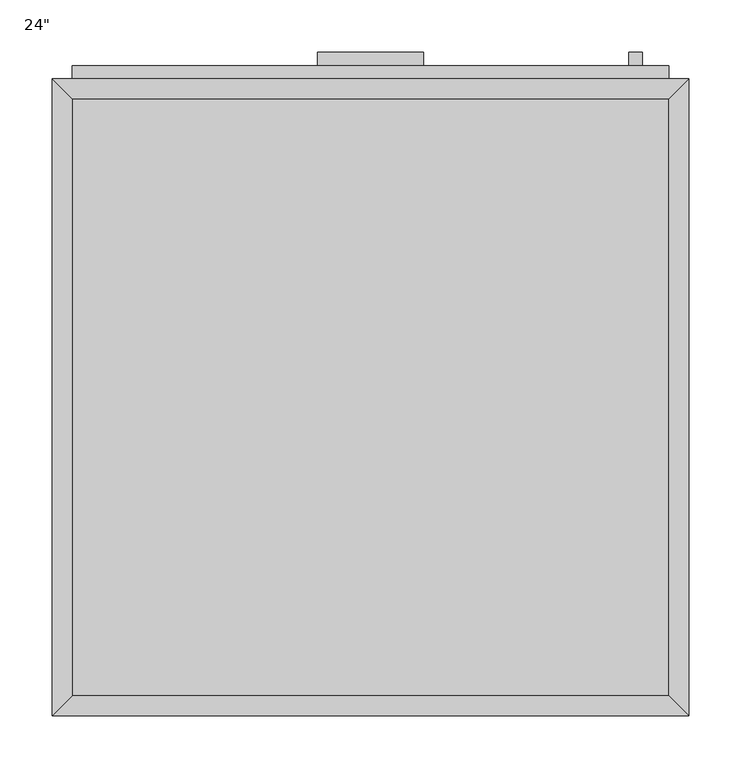
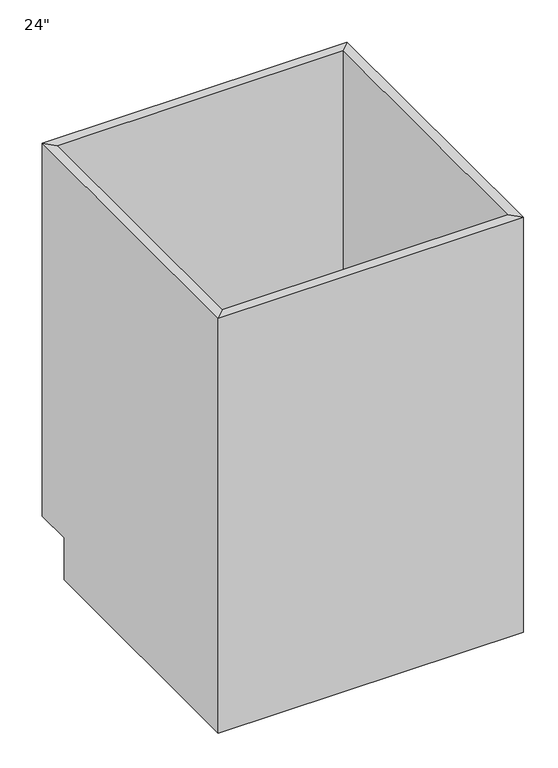
"""IFC4 building model written with IfcOpenShell, lengths in millimetres: furniture geometry."""

from ifc_helpers import new_model, si_unit, frame, origin, place, context, project, spatial, polyline, outline, extrude, faceted_brep, source, transform, mapped, element, save


def furniture_94ff1b7c(model_context):
    return source(origin(), model_context, "Body", "SolidModel", [
        faceted_brep([(304.4877049, 590.55, 876.3), (-267.0122951, 590.55, 876.3), (-267.0122951, 590.55, 88.9), (304.4877049, 590.55, 88.9), (323.5377049, 609.6, 876.3), (-286.0622951, 609.6, 876.3), (323.5377049, 609.6, 88.9), (-286.0622951, 609.6, 88.9), (-267.0122951, 19.05, 876.3), (-267.0122951, 19.05, 88.9), (-267.0122951, 533.4, 88.9), (-286.0622951, 0.0, 876.3), (-286.0622951, 533.4, 88.9), (-286.0622951, 533.4, 0.0), (-286.0622951, 0.0, 0.0), (304.4877049, 19.05, 876.3), (304.4877049, 19.05, 88.9), (323.5377049, 0.0, 876.3), (323.5377049, 0.0, 0.0), (304.4877049, 533.4, 88.9), (323.5377049, 533.4, 0.0), (323.5377049, 533.4, 88.9)], [[[0, 1, 2, 3]], [[0, 4, 5, 1]], [[4, 6, 7, 5]], [[2, 7, 6, 3]], [[1, 8, 9, 10, 2]], [[5, 11, 8, 1]], [[7, 12, 13, 14, 11, 5]], [[2, 10, 12, 7]], [[8, 15, 16, 9]], [[11, 17, 15, 8]], [[14, 18, 17, 11]], [[3, 19, 16, 15, 0]], [[0, 15, 17, 4]], [[4, 17, 18, 20, 21, 6]], [[6, 21, 19, 3]], [[10, 9, 16, 19]], [[18, 14, 13, 20]], [[13, 12, 10, 19, 21, 20]]]),
        extrude(outline(polyline([(279.0877049, 635.0), (279.0877049, 622.3), (266.3877049, 622.3), (266.3877049, 635.0), (279.0877049, 635.0)])), frame((0.0, 0.0, 596.9), z_axis=(0.0, 0.0, 1.0), x_axis=(1.0, 0.0, 0.0)), (0.0, 0.0, 1.0), 101.6),
        extrude(outline(polyline([(69.5377049, 635.0), (69.5377049, 622.3), (-32.0622951, 622.3), (-32.0622951, 635.0), (69.5377049, 635.0)])), frame((0.0, 0.0, 819.15), z_axis=(0.0, 0.0, 1.0), x_axis=(1.0, 0.0, 0.0)), (0.0, 0.0, 1.0), 12.7),
        extrude(outline(polyline([(304.4877049, 622.3), (304.4877049, 609.6), (-267.0122951, 609.6), (-267.0122951, 622.3), (304.4877049, 622.3)])), frame((0.0, 0.0, 107.95), z_axis=(0.0, 0.0, 1.0), x_axis=(1.0, 0.0, 0.0)), (0.0, 0.0, 1.0), 628.65),
        extrude(outline(polyline([(304.4877049, 622.3), (304.4877049, 609.6), (-267.0122951, 609.6), (-267.0122951, 622.3), (304.4877049, 622.3)])), frame((0.0, 0.0, 755.65), z_axis=(0.0, 0.0, 1.0), x_axis=(1.0, 0.0, 0.0)), (0.0, 0.0, 1.0), 101.6),
        extrude(outline(polyline([(304.4877049, 19.05), (-267.0122951, 19.05), (-267.0122951, 590.55), (304.4877049, 590.55), (304.4877049, 19.05)])), frame((0.0, 0.0, 88.9), z_axis=(0.0, 0.0, 1.0), x_axis=(1.0, 0.0, 0.0)), (0.0, 0.0, 1.0), 19.05),
    ])


if __name__ == "__main__":
    model = new_model("IFC4")
    model_context = context("Model", 3, world=origin())
    ifc_project = project(units=[si_unit("LENGTHUNIT", "METRE", prefix="MILLI")], contexts=[model_context])
    site = spatial("IfcSite", under=ifc_project)
    building = spatial("IfcBuilding", under=site)
    placement = place(None, origin())
    furniture_shape = furniture_94ff1b7c(model_context)
    element("IfcFurniture", 1, ObjectType="Base Cabinet-Single Door & Drawer : 24\"", at=placement, inside=building, context=model_context, shape_type="MappedRepresentation", body=[
        mapped(furniture_shape, transform((0.0, 0.0, 0.0), x_axis=(1.0, 0.0, 0.0), y_axis=(0.0, 1.0, 0.0), z_axis=(0.0, 0.0, 1.0))),
    ])
    save(model, "model.ifc")

# Revit data of these elements
# Type "Base Cabinet-Single Door & Drawer : 24\""
#   Assembly Code = "C1030410"
#   Depth = 2' - 0"
#   Height = 2' - 10 1/2"
#   Toe Depth = 0' - 3"
#   Toe Height = 0' - 3 1/2"
#   Width = 2' - 0"
#   Cabinet Material = none
#   Drawer Material = none
#   Handle Material = Cabinets - Handles
#   Default Elevation = 0
# Element 1 (IfcFurniture, "Base Cabinet-Single Door & Drawer : 24\"")
#   Materials on its faces: "Cabinets", "Cabinets - Handles"
# Materials
#   "Cabinets - Handles": class "Unassigned", colour RGB 57 57 57, transparency 0
#   "Cabinets": class "Unassigned", colour RGB 249 249 249, transparency 0
